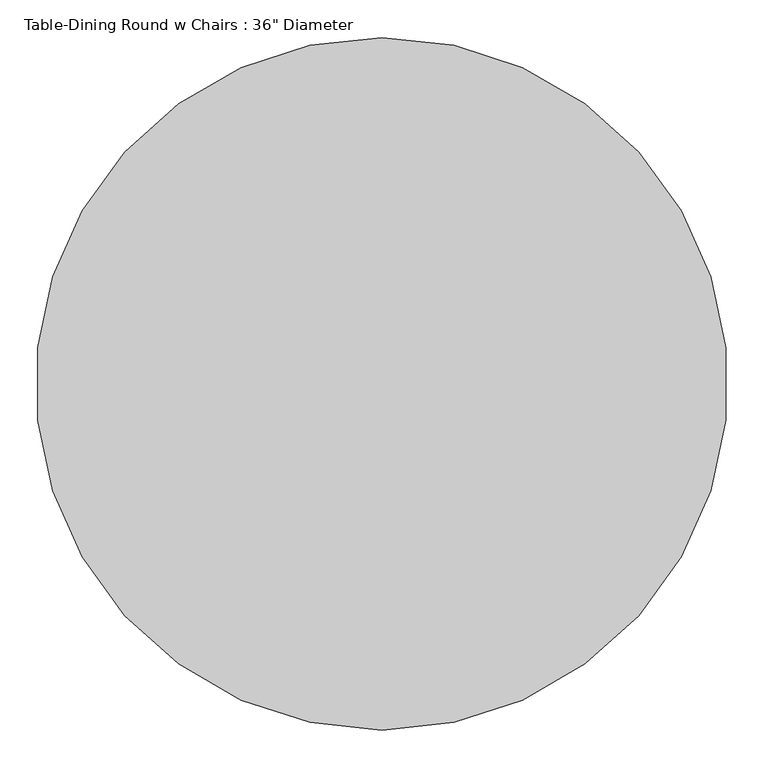
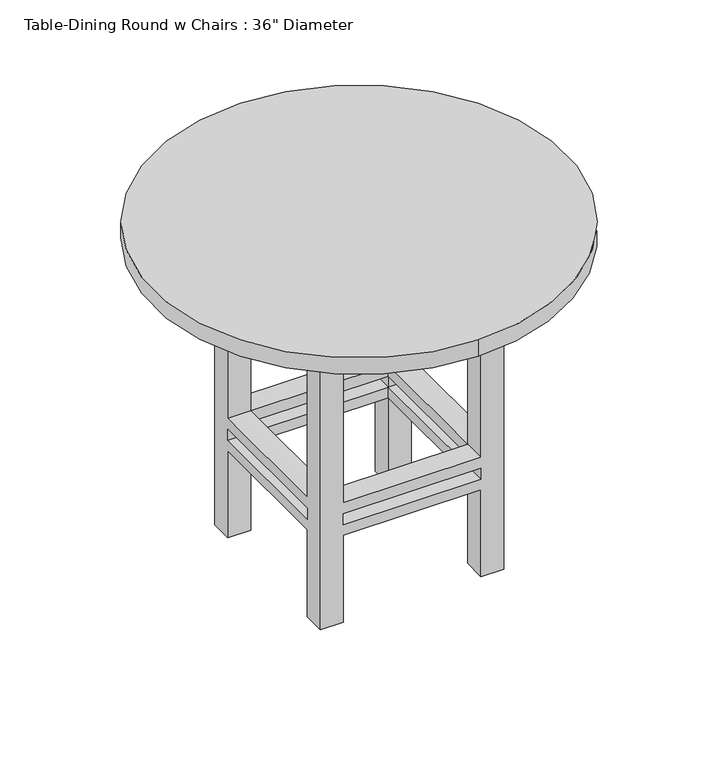
"""IFC4 building model written with IfcOpenShell, lengths in millimetres: furniture geometry."""

from ifc_helpers import new_model, si_unit, point, frame, frame_2d, origin, place, context, project, spatial, polyline, circle_curve, trimmed, segment, composite_curve, outline, extrude, faceted_brep, source, transform, mapped, element, save


def furniture_f004630c(model_context):
    return source(origin(), model_context, "Body", "SolidModel", [
        faceted_brep([(256.0819672, -32.4786885, 279.4), (256.0819672, -337.2786885, 279.4), (306.8819672, -337.2786885, 279.4), (306.8819672, -32.4786885, 279.4), (-48.7180328, -337.2786885, 279.4), (-48.7180328, -388.0786885, 279.4), (256.0819672, -388.0786885, 279.4), (-48.7180328, -32.4786885, 279.4), (-99.5180328, -32.4786885, 279.4), (-99.5180328, -337.2786885, 279.4), (256.0819672, 18.3213115, 279.4), (-48.7180328, 18.3213115, 279.4), (256.0819672, -32.4786885, 254.0), (-48.7180328, -32.4786885, 254.0), (-48.7180328, 18.3213115, 254.0), (256.0819672, 18.3213115, 254.0), (-48.7180328, -337.2786885, 254.0), (-99.5180328, -337.2786885, 254.0), (-99.5180328, -32.4786885, 254.0), (256.0819672, -337.2786885, 254.0), (256.0819672, -388.0786885, 254.0), (-48.7180328, -388.0786885, 254.0), (306.8819672, -32.4786885, 254.0), (306.8819672, -337.2786885, 254.0), (-99.5180328, 18.3213115, 647.7), (-48.7180328, 18.3213115, 647.7), (256.0819672, 18.3213115, 647.7), (306.8819672, 18.3213115, 647.7), (306.8819672, 18.3213115, 0.0), (256.0819672, 18.3213115, 0.0), (256.0819672, 18.3213115, 203.2), (-48.7180328, 18.3213115, 203.2), (-48.7180328, 18.3213115, 0.0), (-99.5180328, 18.3213115, 0.0), (-48.7180328, 18.3213115, 228.6), (256.0819672, 18.3213115, 228.6), (-99.5180328, -32.4786885, 647.7), (-99.5180328, -32.4786885, 0.0), (-99.5180328, -32.4786885, 203.2), (-99.5180328, -337.2786885, 203.2), (-99.5180328, -337.2786885, 0.0), (-99.5180328, -388.0786885, 0.0), (-99.5180328, -388.0786885, 647.7), (-99.5180328, -337.2786885, 647.7), (-99.5180328, -337.2786885, 228.6), (-99.5180328, -32.4786885, 228.6), (306.8819672, -388.0786885, 647.7), (256.0819672, -388.0786885, 647.7), (-48.7180328, -388.0786885, 647.7), (-48.7180328, -388.0786885, 0.0), (-48.7180328, -388.0786885, 203.2), (256.0819672, -388.0786885, 203.2), (256.0819672, -388.0786885, 0.0), (306.8819672, -388.0786885, 0.0), (256.0819672, -388.0786885, 228.6), (-48.7180328, -388.0786885, 228.6), (306.8819672, -32.4786885, 647.7), (306.8819672, -337.2786885, 647.7), (306.8819672, -337.2786885, 0.0), (306.8819672, -337.2786885, 203.2), (306.8819672, -32.4786885, 203.2), (306.8819672, -32.4786885, 0.0), (306.8819672, -32.4786885, 228.6), (306.8819672, -337.2786885, 228.6), (-48.7180328, -32.4786885, 647.7), (256.0819672, -32.4786885, 647.7), (256.0819672, -337.2786885, 647.7), (-48.7180328, -337.2786885, 647.7), (-48.7180328, -32.4786885, 0.0), (256.0819672, -32.4786885, 0.0), (256.0819672, -337.2786885, 0.0), (-48.7180328, -337.2786885, 0.0), (-48.7180328, -32.4786885, 203.2), (-48.7180328, -32.4786885, 228.6), (256.0819672, -32.4786885, 203.2), (256.0819672, -32.4786885, 228.6), (256.0819672, -337.2786885, 203.2), (256.0819672, -337.2786885, 228.6), (-48.7180328, -337.2786885, 203.2), (-48.7180328, -337.2786885, 228.6)], [[[0, 1, 2, 3]], [[1, 4, 5, 6]], [[4, 7, 8, 9]], [[7, 0, 10, 11]], [[12, 13, 14, 15]], [[13, 16, 17, 18]], [[16, 19, 20, 21]], [[19, 12, 22, 23]], [[24, 25, 11, 10, 26, 27, 28, 29, 30, 31, 32, 33], [14, 34, 35, 15]], [[36, 24, 33, 37, 38, 39, 40, 41, 42, 43, 9, 8], [17, 44, 45, 18]], [[46, 47, 6, 5, 48, 42, 41, 49, 50, 51, 52, 53], [20, 54, 55, 21]], [[28, 27, 56, 3, 2, 57, 46, 53, 58, 59, 60, 61], [22, 62, 63, 23]], [[1, 0, 12, 19]], [[4, 1, 19, 16]], [[7, 4, 16, 13]], [[0, 7, 13, 12]], [[25, 24, 36, 64]], [[26, 65, 56, 27]], [[47, 46, 57, 66]], [[48, 67, 43, 42]], [[32, 68, 37, 33]], [[29, 28, 61, 69]], [[52, 70, 58, 53]], [[49, 41, 40, 71]], [[64, 36, 8, 7]], [[37, 68, 72, 38]], [[13, 18, 45, 73]], [[25, 64, 7, 11]], [[68, 32, 31, 72]], [[14, 13, 73, 34]], [[65, 26, 10, 0]], [[29, 69, 74, 30]], [[12, 15, 35, 75]], [[56, 65, 0, 3]], [[69, 61, 60, 74]], [[22, 12, 75, 62]], [[66, 57, 2, 1]], [[58, 70, 76, 59]], [[19, 23, 63, 77]], [[47, 66, 1, 6]], [[70, 52, 51, 76]], [[20, 19, 77, 54]], [[67, 48, 5, 4]], [[49, 71, 78, 50]], [[16, 21, 55, 79]], [[43, 67, 4, 9]], [[71, 40, 39, 78]], [[17, 16, 79, 44]], [[75, 77, 63, 62]], [[77, 79, 55, 54]], [[79, 73, 45, 44]], [[73, 75, 35, 34]], [[74, 72, 31, 30]], [[72, 78, 39, 38]], [[78, 76, 51, 50]], [[76, 74, 60, 59]], [[77, 75, 74, 76]], [[79, 77, 76, 78]], [[73, 79, 78, 72]], [[75, 73, 72, 74]]]),
        extrude(outline(polyline([(332.2819672, 43.7213115), (332.2819672, -413.4786885), (-124.9180328, -413.4786885), (-124.9180328, 43.7213115), (332.2819672, 43.7213115)]), holes=[polyline([(306.8819672, 18.3213115), (-99.5180328, 18.3213115), (-99.5180328, -388.0786885), (306.8819672, -388.0786885), (306.8819672, 18.3213115)])]), frame((0.0, 0.0, 647.7), z_axis=(0.0, 0.0, 1.0), x_axis=(1.0, 0.0, 0.0)), (0.0, 0.0, 1.0), 76.2),
        extrude(outline(composite_curve([segment(trimmed(circle_curve(frame_2d((103.6819672, -184.8786885)), 457.2), [point((103.6819672, -642.0786885))], [point((103.6819672, 272.3213115))], False, "CARTESIAN"), True, "CONTINUOUS"), segment(trimmed(circle_curve(frame_2d((103.6819672, -184.8786885)), 457.2), [point((103.6819672, 272.3213115))], [point((103.6819672, -642.0786885))], False, "CARTESIAN"), True, "CONTINUOUS")], self_intersect=False)), frame((0.0, 0.0, 723.9), z_axis=(0.0, 0.0, 1.0), x_axis=(1.0, 0.0, 0.0)), (0.0, 0.0, 1.0), 38.1),
    ])


if __name__ == "__main__":
    model = new_model("IFC4")
    model_context = context("Model", 3, world=origin())
    ifc_project = project(units=[si_unit("LENGTHUNIT", "METRE", prefix="MILLI")], contexts=[model_context])
    site = spatial("IfcSite", under=ifc_project)
    building = spatial("IfcBuilding", under=site)
    placement = place(None, origin())
    furniture_shape = furniture_f004630c(model_context)
    element("IfcFurniture", 1, ObjectType="Table-Dining Round w Chairs : 36\" Diameter", at=placement, inside=building, context=model_context, shape_type="MappedRepresentation", body=[
        mapped(furniture_shape, transform((0.0, 0.0, 0.0), x_axis=(1.0, 0.0, 0.0), y_axis=(0.0, 1.0, 0.0), z_axis=(0.0, 0.0, 1.0))),
    ])
    save(model, "model.ifc")

# Revit data of these elements
# Type "Table-Dining Round w Chairs : 36\" Diameter"
#   Assembly Code = "E2020200"
#   Cost = 300
#   Radius = 1' - 6"
#   Diameter = 3' - 0"
#   Height = 2' - 6"
#   Chairs = 4
#   Base Material = Wood - Pine
#   Top Material = Laminate - Linen, Matte
# Element 1 (IfcFurniture, "Table-Dining Round w Chairs : 36\" Diameter")
#   Materials on its faces: "Wood - Pine", "Laminate - Linen, Matte"
# Materials
#   "Wood - Pine": class "Wood", colour RGB 223 192 134, transparency 0
#   "Laminate - Linen, Matte": class "Miscellaneous", colour RGB 249 239 230, transparency 0
